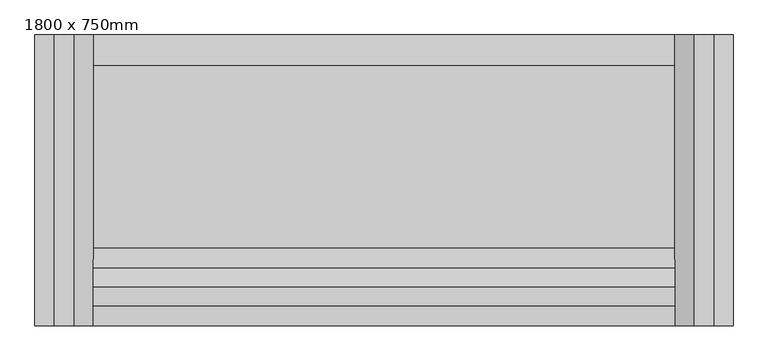
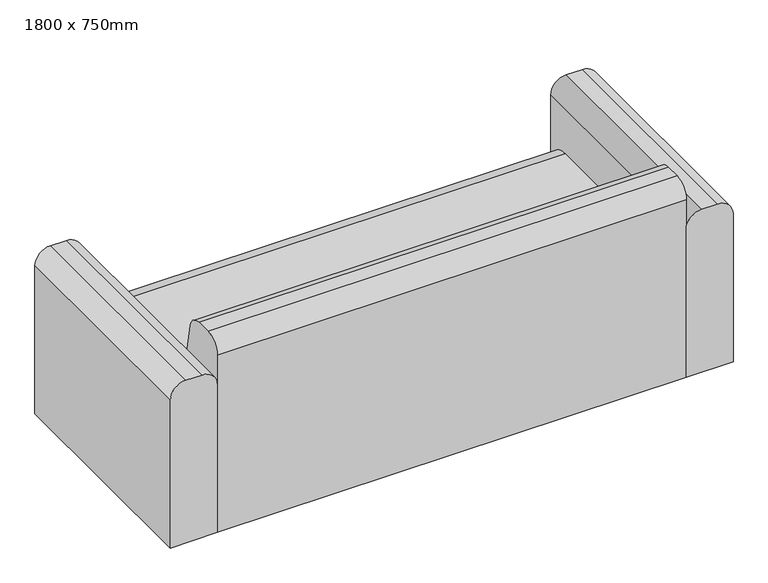
"""IFC4 building model written with IfcOpenShell, lengths in millimetres: furniture geometry, ソファ－I型 : 1800 x 750mm."""

import ifcopenshell
import ifcopenshell.guid

model = None  # the IFC model being written
_history = None  # IfcOwnerHistory: only IFC2X3 demands one
_inside = {}  # id of a spatial element -> (the spatial element, [elements in it])
_under = {}  # id of a project, library or spatial element -> (it, [spatial elements below it])
_declared = {}  # id of a project -> (the project, [libraries it declares])
_typed = {}  # id of a type object -> (the type object, [elements of that type])
_made_of = {}  # id of a material, layer set ... -> (it, [elements and type objects made of it])


def new_model(schema):
    """Start an empty IFC model of exactly this schema.

    Asked for "IFC4X3", IfcOpenShell would pick the latest addendum, in which some entities
    have other attributes; the version numbers below select the first issue.
    IFC2X3 requires an IfcOwnerHistory on every rooted entity: one is made here for all.
    """
    global model, _history
    if schema == "IFC4X3":
        model = ifcopenshell.file(schema_version=(4, 3, 0, 0))
    else:
        model = ifcopenshell.file(schema=schema)
    _inside.clear()
    _under.clear()
    _declared.clear()
    _typed.clear()
    _made_of.clear()
    _history = None
    if model.schema == "IFC2X3":
        org = make("IfcOrganization", Name="unknown")
        user = make(
            "IfcPersonAndOrganization",
            ThePerson=make("IfcPerson", FamilyName="unknown"),
            TheOrganization=org,
        )
        app = make(
            "IfcApplication",
            ApplicationDeveloper=org,
            Version="unknown",
            ApplicationFullName="unknown",
            ApplicationIdentifier="unknown",
        )
        _history = make(
            "IfcOwnerHistory",
            OwningUser=user,
            OwningApplication=app,
            ChangeAction="ADDED",
            CreationDate=0,
        )
    return model


def make(cls, **values):
    """One entity of the class cls with the attributes given. An attribute that is None is left unset."""
    return model.create_entity(
        cls, **{name: value for name, value in values.items() if value is not None}
    )


def rooted(cls, **values):
    """An entity with a GlobalId (a new one), such as an element, a storey or a relation."""
    return make(cls, GlobalId=ifcopenshell.guid.new(), OwnerHistory=_history, **values)


def si_unit(unit_type, name, prefix=None):
    """IfcSIUnit, for example si_unit("LENGTHUNIT", "METRE", prefix="MILLI")."""
    return make("IfcSIUnit", UnitType=unit_type, Prefix=prefix, Name=name)


def assignment(units):
    """IfcUnitAssignment: the units of a project."""
    return None if units is None else make("IfcUnitAssignment", Units=units)


def point(xyz):
    """IfcCartesianPoint."""
    return None if xyz is None else make("IfcCartesianPoint", Coordinates=xyz)


def direction(xyz):
    """IfcDirection."""
    return None if xyz is None else make("IfcDirection", DirectionRatios=xyz)


def frame(location, z_axis=None, x_axis=None):
    """IfcAxis2Placement3D, a coordinate frame: its origin and axes. An axis left out is left unset."""
    return make(
        "IfcAxis2Placement3D",
        Location=point(location),
        Axis=direction(z_axis),
        RefDirection=direction(x_axis),
    )


def frame_2d(location, x_axis=None):
    """IfcAxis2Placement2D, a coordinate frame in the plane: its origin and x axis."""
    return make(
        "IfcAxis2Placement2D", Location=point(location), RefDirection=direction(x_axis)
    )


def origin():
    """The frame at (0, 0, 0) with its axes left unset."""
    return frame((0.0, 0.0, 0.0))


def place(relative_to, where):
    """IfcLocalPlacement: puts the frame where relative to a parent placement (None: the world)."""
    return make(
        "IfcLocalPlacement", PlacementRelTo=relative_to, RelativePlacement=where
    )


def context(
    kind, dimensions, precision=None, world=None, true_north=None, identifier=None
):
    """IfcGeometricRepresentationContext, for example the 3D "Model" context."""
    return make(
        "IfcGeometricRepresentationContext",
        ContextIdentifier=identifier,
        ContextType=kind,
        CoordinateSpaceDimension=dimensions,
        Precision=precision,
        WorldCoordinateSystem=world,
        TrueNorth=true_north,
    )


def project(units=None, contexts=None):
    """IfcProject with its units and contexts."""
    return rooted(
        "IfcProject",
        Name="project",
        RepresentationContexts=contexts,
        UnitsInContext=assignment(units),
    )


def spatial(cls, under=None, at=None, **own):
    """A site, building, storey or space (cls), placed at a placement, below another one or the project."""
    s = rooted(cls, ObjectPlacement=at, **own)
    if under is not None:
        _under.setdefault(under.id(), (under, []))[1].append(s)
    return s


def polyline(points):
    """IfcPolyline through the points."""
    return make("IfcPolyline", Points=[point(p) for p in points])


def circle_curve(where, radius):
    """IfcCircle in the frame where."""
    return make("IfcCircle", Position=where, Radius=radius)


def trimmed(basis, trim1, trim2, sense, master):
    """IfcTrimmedCurve: the piece of a basis curve between two trims."""
    return make(
        "IfcTrimmedCurve",
        BasisCurve=basis,
        Trim1=trim1,
        Trim2=trim2,
        SenseAgreement=sense,
        MasterRepresentation=master,
    )


def segment(curve, same_sense, transition):
    """IfcCompositeCurveSegment."""
    return make(
        "IfcCompositeCurveSegment",
        Transition=transition,
        SameSense=same_sense,
        ParentCurve=curve,
    )


def composite_curve(segments, self_intersect=None):
    """IfcCompositeCurve: segments joined end to end."""
    return make("IfcCompositeCurve", Segments=segments, SelfIntersect=self_intersect)


def outline(outer, holes=None, kind="AREA"):
    """IfcArbitraryClosedProfileDef: a profile drawn as a closed curve; with holes, ...WithVoids."""
    if holes is None:
        return make("IfcArbitraryClosedProfileDef", ProfileType=kind, OuterCurve=outer)
    return make(
        "IfcArbitraryProfileDefWithVoids",
        ProfileType=kind,
        OuterCurve=outer,
        InnerCurves=holes,
    )


def extrude(swept, where, along, depth):
    """IfcExtrudedAreaSolid: the profile swept, set in the frame where, extruded along a direction by depth."""
    return make(
        "IfcExtrudedAreaSolid",
        SweptArea=swept,
        Position=where,
        ExtrudedDirection=direction(along),
        Depth=depth,
    )


def shape(context_of_items, identifier, shape_type, items):
    """IfcShapeRepresentation: the items that make up one representation, for example the "Body"."""
    return make(
        "IfcShapeRepresentation",
        ContextOfItems=context_of_items,
        RepresentationIdentifier=identifier,
        RepresentationType=shape_type,
        Items=items,
    )


def source(mapping_origin, context_of_items, identifier, shape_type, items):
    """IfcRepresentationMap: a shape defined once, which mapped items show again and again."""
    return make(
        "IfcRepresentationMap",
        MappingOrigin=mapping_origin,
        MappedRepresentation=shape(context_of_items, identifier, shape_type, items),
    )


def transform(
    local_origin,
    x_axis=None,
    y_axis=None,
    z_axis=None,
    scale=None,
    scale2=None,
    scale3=None,
    uniform=True,
):
    """IfcCartesianTransformationOperator3D, or its non-uniform kind. x_axis, y_axis, z_axis: its Axis1, 2, 3."""
    if uniform:
        return make(
            "IfcCartesianTransformationOperator3D",
            Axis1=direction(x_axis),
            Axis2=direction(y_axis),
            LocalOrigin=point(local_origin),
            Scale=scale,
            Axis3=direction(z_axis),
        )
    return make(
        "IfcCartesianTransformationOperator3DnonUniform",
        Axis1=direction(x_axis),
        Axis2=direction(y_axis),
        LocalOrigin=point(local_origin),
        Scale=scale,
        Axis3=direction(z_axis),
        Scale2=scale2,
        Scale3=scale3,
    )


def mapped(mapping_source, mapping_target):
    """IfcMappedItem: shows the shape of a source again, moved by a transform."""
    return make(
        "IfcMappedItem", MappingSource=mapping_source, MappingTarget=mapping_target
    )


def made_of(thing, what):
    """Note that an element or type object is made of a material, layer set ...; save() writes the relation."""
    if what is not None:
        _made_of.setdefault(what.id(), (what, []))[1].append(thing)
    return thing


def element(
    cls,
    number,
    at=None,
    inside=None,
    cuts=None,
    type_object=None,
    material=None,
    context=None,
    identifier="Body",
    shape_type=None,
    held_by="IfcProductDefinitionShape",
    body=None,
    shapes=None,
    **own,
):
    """One element of the class cls, such as IfcWall. Its Tag is "e" and its number.

    at: its placement. inside: the storey or other place that contains it. cuts: it is an
    opening in that element (IfcRelVoidsElement). A single representation is given by context,
    identifier, shape_type and body (its items); several are given by shapes. held_by: the class
    of the entity that holds the representations. save() writes the other relations.
    """
    e = rooted(cls, Tag="e%d" % number, ObjectPlacement=at, **own)
    if body is not None:
        shapes = [shape(context, identifier, shape_type, body)]
    if shapes is not None:
        e.Representation = make(held_by, Representations=shapes)
    if inside is not None:
        _inside.setdefault(inside.id(), (inside, []))[1].append(e)
    if cuts is not None:
        rooted(
            "IfcRelVoidsElement", RelatingBuildingElement=cuts, RelatedOpeningElement=e
        )
    if type_object is not None:
        _typed.setdefault(type_object.id(), (type_object, []))[1].append(e)
    return made_of(e, material)


def aggregate(whole, parts):
    """IfcRelAggregates: a whole, such as a stair, and the parts it consists of."""
    return rooted("IfcRelAggregates", RelatingObject=whole, RelatedObjects=parts)


def save(model, path):
    """Write the relations noted so far, then the file.

    IfcRelAggregates (storeys below a building ...), IfcRelContainedInSpatialStructure (elements
    in a storey), IfcRelDefinesByType, IfcRelAssociatesMaterial and IfcRelDeclares: one each for
    every whole, place, type object, material and project.
    """
    for whole, parts in _under.values():
        aggregate(whole, parts)
    for where, things in _inside.values():
        rooted(
            "IfcRelContainedInSpatialStructure",
            RelatedElements=things,
            RelatingStructure=where,
        )
    for kind, things in _typed.values():
        rooted("IfcRelDefinesByType", RelatedObjects=things, RelatingType=kind)
    for what, things in _made_of.values():
        rooted("IfcRelAssociatesMaterial", RelatedObjects=things, RelatingMaterial=what)
    for by, libraries in _declared.values():
        rooted("IfcRelDeclares", RelatingContext=by, RelatedDefinitions=libraries)
    model.write(path)


def furniture_1800_x_750mm_5b3da114(model_context):
    return source(origin(), model_context, "Body", "SweptSolid", [
        extrude(outline(composite_curve([segment(trimmed(circle_curve(frame_2d((500.0, -850.0)), 50.0), [point((550.0, -850.0))], [point((500.0, -900.0))], False, "CARTESIAN"), True, "CONTINUOUS"), segment(polyline([(500.0, -900.0), (0.0, -900.0), (0.0, -750.0), (500.0, -750.0)]), True, "CONTINUOUS"), segment(trimmed(circle_curve(frame_2d((500.0, -800.0)), 50.0), [point((500.0, -750.0))], [point((550.0, -800.0))], False, "CARTESIAN"), True, "CONTINUOUS"), segment(polyline([(550.0, -800.0), (550.0, -850.0)]), True, "CONTINUOUS")], self_intersect=False)), frame((0.0, -375.0, 0.0), z_axis=(0.0, 1.0, 0.0), x_axis=(0.0, 0.0, 1.0)), (0.0, 0.0, 1.0), 750.0),
        extrude(outline(composite_curve([segment(polyline([(550.0, 850.0), (550.0, 800.0)]), True, "CONTINUOUS"), segment(trimmed(circle_curve(frame_2d((500.0, 800.0)), 50.0), [point((550.0, 800.0))], [point((500.0, 750.0))], False, "CARTESIAN"), True, "CONTINUOUS"), segment(polyline([(500.0, 750.0), (0.0, 750.0), (0.0, 900.0), (500.0, 900.0)]), True, "CONTINUOUS"), segment(trimmed(circle_curve(frame_2d((500.0, 850.0)), 50.0), [point((500.0, 900.0))], [point((550.0, 850.0))], False, "CARTESIAN"), True, "CONTINUOUS")], self_intersect=False)), frame((0.0, -375.0, 0.0), z_axis=(0.0, 1.0, 0.0), x_axis=(0.0, 0.0, 1.0)), (0.0, 0.0, 1.0), 750.0),
        extrude(outline(composite_curve([segment(polyline([(-226.9611614, 609.8058068), (-175.0, 350.0), (295.0, 350.0)]), True, "CONTINUOUS"), segment(trimmed(circle_curve(frame_2d((295.0, 270.0)), 80.0), [point((295.0, 350.0))], [point((375.0, 270.0))], False, "CARTESIAN"), True, "CONTINUOUS"), segment(polyline([(375.0, 270.0), (375.0, 60.0), (305.0, 60.0), (305.0, 0.0), (-375.0, 0.0), (-375.0, 600.0)]), True, "CONTINUOUS"), segment(trimmed(circle_curve(frame_2d((-325.0, 600.0)), 50.0), [point((-375.0, 600.0))], [point((-325.0, 650.0))], False, "CARTESIAN"), True, "CONTINUOUS"), segment(polyline([(-325.0, 650.0), (-275.9901951, 650.0)]), True, "CONTINUOUS"), segment(trimmed(circle_curve(frame_2d((-275.9901951, 600.0)), 50.0), [point((-275.9901951, 650.0))], [point((-226.9611614, 609.8058068))], False, "CARTESIAN"), True, "CONTINUOUS")], self_intersect=False)), frame((-750.0, 0.0, 0.0), z_axis=(1.0, 0.0, 0.0), x_axis=(0.0, 1.0, 0.0)), (0.0, 0.0, 1.0), 1500.0),
    ])


if __name__ == "__main__":
    model = new_model("IFC4")
    model_context = context("Model", 3, world=origin())
    ifc_project = project(units=[si_unit("LENGTHUNIT", "METRE", prefix="MILLI")], contexts=[model_context])
    site = spatial("IfcSite", under=ifc_project)
    building = spatial("IfcBuilding", under=site)
    placement = place(None, origin())
    furniture_1800_x_750mm_shape = furniture_1800_x_750mm_5b3da114(model_context)
    element("IfcFurniture", 1, ObjectType="ソファ－I型 : 1800 x 750mm", at=placement, inside=building, context=model_context, shape_type="MappedRepresentation", body=[
        mapped(furniture_1800_x_750mm_shape, transform((0.0, 0.0, 0.0), x_axis=(1.0, 0.0, 0.0), y_axis=(0.0, 1.0, 0.0), z_axis=(0.0, 0.0, 1.0))),
    ])
    save(model, "model.ifc")

# Revit data of these elements
# Type "ソファ－I型 : 1800 x 750mm"
#   Keynote = "12490.Y1"
#   座面高さ = 350 mm
#   幅 = 1800 mm
#   奥行き = 750 mm
#   本体 = モチアミ - 無地 - グレー
#   Default Elevation = 0
# Element 1 (IfcFurniture, "ソファ－I型 : 1800 x 750mm")
#   Materials on its faces: "モチアミ - 無地 - グレー"
# Materials
#   "モチアミ - 無地 - グレー": class "モチアミ", colour RGB 65 63 65, transparency 0, Cost = 0
